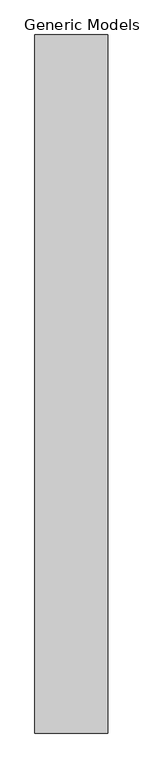
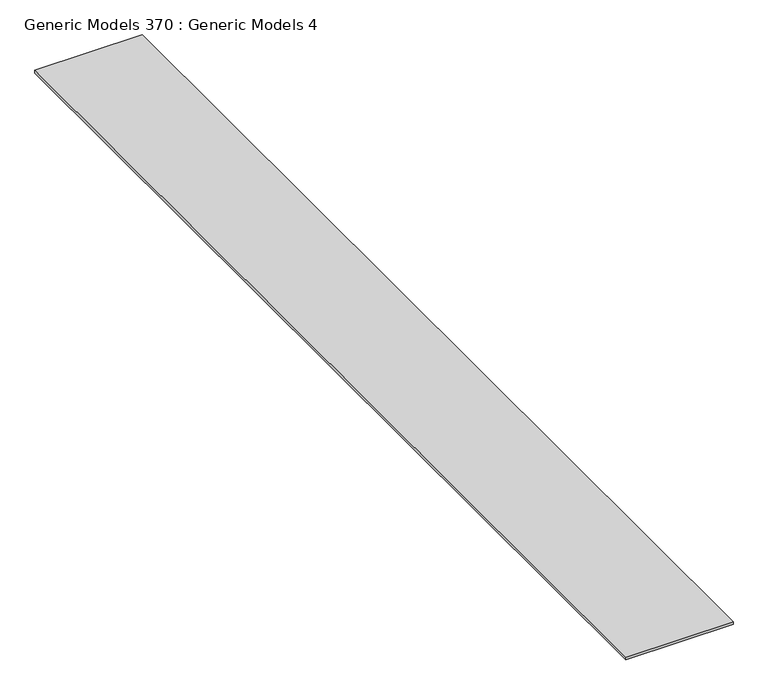
"""IFC4 building model written with IfcOpenShell, lengths in millimetres: proxy geometry, Generic Models 370 : Generic Models 4."""

import ifcopenshell
import ifcopenshell.guid

model = None  # the IFC model being written
_history = None  # IfcOwnerHistory: only IFC2X3 demands one
_inside = {}  # id of a spatial element -> (the spatial element, [elements in it])
_under = {}  # id of a project, library or spatial element -> (it, [spatial elements below it])
_declared = {}  # id of a project -> (the project, [libraries it declares])
_typed = {}  # id of a type object -> (the type object, [elements of that type])
_made_of = {}  # id of a material, layer set ... -> (it, [elements and type objects made of it])


def new_model(schema):
    """Start an empty IFC model of exactly this schema.

    Asked for "IFC4X3", IfcOpenShell would pick the latest addendum, in which some entities
    have other attributes; the version numbers below select the first issue.
    IFC2X3 requires an IfcOwnerHistory on every rooted entity: one is made here for all.
    """
    global model, _history
    if schema == "IFC4X3":
        model = ifcopenshell.file(schema_version=(4, 3, 0, 0))
    else:
        model = ifcopenshell.file(schema=schema)
    _inside.clear()
    _under.clear()
    _declared.clear()
    _typed.clear()
    _made_of.clear()
    _history = None
    if model.schema == "IFC2X3":
        org = make("IfcOrganization", Name="unknown")
        user = make(
            "IfcPersonAndOrganization",
            ThePerson=make("IfcPerson", FamilyName="unknown"),
            TheOrganization=org,
        )
        app = make(
            "IfcApplication",
            ApplicationDeveloper=org,
            Version="unknown",
            ApplicationFullName="unknown",
            ApplicationIdentifier="unknown",
        )
        _history = make(
            "IfcOwnerHistory",
            OwningUser=user,
            OwningApplication=app,
            ChangeAction="ADDED",
            CreationDate=0,
        )
    return model


def make(cls, **values):
    """One entity of the class cls with the attributes given. An attribute that is None is left unset."""
    return model.create_entity(
        cls, **{name: value for name, value in values.items() if value is not None}
    )


def rooted(cls, **values):
    """An entity with a GlobalId (a new one), such as an element, a storey or a relation."""
    return make(cls, GlobalId=ifcopenshell.guid.new(), OwnerHistory=_history, **values)


def si_unit(unit_type, name, prefix=None):
    """IfcSIUnit, for example si_unit("LENGTHUNIT", "METRE", prefix="MILLI")."""
    return make("IfcSIUnit", UnitType=unit_type, Prefix=prefix, Name=name)


def assignment(units):
    """IfcUnitAssignment: the units of a project."""
    return None if units is None else make("IfcUnitAssignment", Units=units)


def point(xyz):
    """IfcCartesianPoint."""
    return None if xyz is None else make("IfcCartesianPoint", Coordinates=xyz)


def direction(xyz):
    """IfcDirection."""
    return None if xyz is None else make("IfcDirection", DirectionRatios=xyz)


def frame(location, z_axis=None, x_axis=None):
    """IfcAxis2Placement3D, a coordinate frame: its origin and axes. An axis left out is left unset."""
    return make(
        "IfcAxis2Placement3D",
        Location=point(location),
        Axis=direction(z_axis),
        RefDirection=direction(x_axis),
    )


def origin():
    """The frame at (0, 0, 0) with its axes left unset."""
    return frame((0.0, 0.0, 0.0))


def place(relative_to, where):
    """IfcLocalPlacement: puts the frame where relative to a parent placement (None: the world)."""
    return make(
        "IfcLocalPlacement", PlacementRelTo=relative_to, RelativePlacement=where
    )


def context(
    kind, dimensions, precision=None, world=None, true_north=None, identifier=None
):
    """IfcGeometricRepresentationContext, for example the 3D "Model" context."""
    return make(
        "IfcGeometricRepresentationContext",
        ContextIdentifier=identifier,
        ContextType=kind,
        CoordinateSpaceDimension=dimensions,
        Precision=precision,
        WorldCoordinateSystem=world,
        TrueNorth=true_north,
    )


def project(units=None, contexts=None):
    """IfcProject with its units and contexts."""
    return rooted(
        "IfcProject",
        Name="project",
        RepresentationContexts=contexts,
        UnitsInContext=assignment(units),
    )


def spatial(cls, under=None, at=None, **own):
    """A site, building, storey or space (cls), placed at a placement, below another one or the project."""
    s = rooted(cls, ObjectPlacement=at, **own)
    if under is not None:
        _under.setdefault(under.id(), (under, []))[1].append(s)
    return s


def polyline(points):
    """IfcPolyline through the points."""
    return make("IfcPolyline", Points=[point(p) for p in points])


def outline(outer, holes=None, kind="AREA"):
    """IfcArbitraryClosedProfileDef: a profile drawn as a closed curve; with holes, ...WithVoids."""
    if holes is None:
        return make("IfcArbitraryClosedProfileDef", ProfileType=kind, OuterCurve=outer)
    return make(
        "IfcArbitraryProfileDefWithVoids",
        ProfileType=kind,
        OuterCurve=outer,
        InnerCurves=holes,
    )


def extrude(swept, where, along, depth):
    """IfcExtrudedAreaSolid: the profile swept, set in the frame where, extruded along a direction by depth."""
    return make(
        "IfcExtrudedAreaSolid",
        SweptArea=swept,
        Position=where,
        ExtrudedDirection=direction(along),
        Depth=depth,
    )


def shape(context_of_items, identifier, shape_type, items):
    """IfcShapeRepresentation: the items that make up one representation, for example the "Body"."""
    return make(
        "IfcShapeRepresentation",
        ContextOfItems=context_of_items,
        RepresentationIdentifier=identifier,
        RepresentationType=shape_type,
        Items=items,
    )


def source(mapping_origin, context_of_items, identifier, shape_type, items):
    """IfcRepresentationMap: a shape defined once, which mapped items show again and again."""
    return make(
        "IfcRepresentationMap",
        MappingOrigin=mapping_origin,
        MappedRepresentation=shape(context_of_items, identifier, shape_type, items),
    )


def transform(
    local_origin,
    x_axis=None,
    y_axis=None,
    z_axis=None,
    scale=None,
    scale2=None,
    scale3=None,
    uniform=True,
):
    """IfcCartesianTransformationOperator3D, or its non-uniform kind. x_axis, y_axis, z_axis: its Axis1, 2, 3."""
    if uniform:
        return make(
            "IfcCartesianTransformationOperator3D",
            Axis1=direction(x_axis),
            Axis2=direction(y_axis),
            LocalOrigin=point(local_origin),
            Scale=scale,
            Axis3=direction(z_axis),
        )
    return make(
        "IfcCartesianTransformationOperator3DnonUniform",
        Axis1=direction(x_axis),
        Axis2=direction(y_axis),
        LocalOrigin=point(local_origin),
        Scale=scale,
        Axis3=direction(z_axis),
        Scale2=scale2,
        Scale3=scale3,
    )


def mapped(mapping_source, mapping_target):
    """IfcMappedItem: shows the shape of a source again, moved by a transform."""
    return make(
        "IfcMappedItem", MappingSource=mapping_source, MappingTarget=mapping_target
    )


def made_of(thing, what):
    """Note that an element or type object is made of a material, layer set ...; save() writes the relation."""
    if what is not None:
        _made_of.setdefault(what.id(), (what, []))[1].append(thing)
    return thing


def element(
    cls,
    number,
    at=None,
    inside=None,
    cuts=None,
    type_object=None,
    material=None,
    context=None,
    identifier="Body",
    shape_type=None,
    held_by="IfcProductDefinitionShape",
    body=None,
    shapes=None,
    **own,
):
    """One element of the class cls, such as IfcWall. Its Tag is "e" and its number.

    at: its placement. inside: the storey or other place that contains it. cuts: it is an
    opening in that element (IfcRelVoidsElement). A single representation is given by context,
    identifier, shape_type and body (its items); several are given by shapes. held_by: the class
    of the entity that holds the representations. save() writes the other relations.
    """
    e = rooted(cls, Tag="e%d" % number, ObjectPlacement=at, **own)
    if body is not None:
        shapes = [shape(context, identifier, shape_type, body)]
    if shapes is not None:
        e.Representation = make(held_by, Representations=shapes)
    if inside is not None:
        _inside.setdefault(inside.id(), (inside, []))[1].append(e)
    if cuts is not None:
        rooted(
            "IfcRelVoidsElement", RelatingBuildingElement=cuts, RelatedOpeningElement=e
        )
    if type_object is not None:
        _typed.setdefault(type_object.id(), (type_object, []))[1].append(e)
    return made_of(e, material)


def aggregate(whole, parts):
    """IfcRelAggregates: a whole, such as a stair, and the parts it consists of."""
    return rooted("IfcRelAggregates", RelatingObject=whole, RelatedObjects=parts)


def save(model, path):
    """Write the relations noted so far, then the file.

    IfcRelAggregates (storeys below a building ...), IfcRelContainedInSpatialStructure (elements
    in a storey), IfcRelDefinesByType, IfcRelAssociatesMaterial and IfcRelDeclares: one each for
    every whole, place, type object, material and project.
    """
    for whole, parts in _under.values():
        aggregate(whole, parts)
    for where, things in _inside.values():
        rooted(
            "IfcRelContainedInSpatialStructure",
            RelatedElements=things,
            RelatingStructure=where,
        )
    for kind, things in _typed.values():
        rooted("IfcRelDefinesByType", RelatedObjects=things, RelatingType=kind)
    for what, things in _made_of.values():
        rooted("IfcRelAssociatesMaterial", RelatedObjects=things, RelatingMaterial=what)
    for by, libraries in _declared.values():
        rooted("IfcRelDeclares", RelatingContext=by, RelatedDefinitions=libraries)
    model.write(path)


def generic_models_370_generic_models_4_c4932353(model_context):
    return source(origin(), model_context, "Body", "SweptSolid", [
        extrude(outline(polyline([(10201.955181, -6864.9230338), (9532.1363263, -6864.9230338), (9532.1363263, -464.1230338), (10201.955181, -464.1230338), (10201.955181, -6864.9230338)])), frame((0.0, 0.0, 128179.3644528), z_axis=(0.0, 0.0, 1.0), x_axis=(1.0, 0.0, 0.0)), (0.0, 0.0, 1.0), 19.05),
    ])


if __name__ == "__main__":
    model = new_model("IFC4")
    model_context = context("Model", 3, world=origin())
    ifc_project = project(units=[si_unit("LENGTHUNIT", "METRE", prefix="MILLI")], contexts=[model_context])
    site = spatial("IfcSite", under=ifc_project)
    building = spatial("IfcBuilding", under=site)
    placement = place(None, origin())
    generic_models_370_generic_models_4_shape = generic_models_370_generic_models_4_c4932353(model_context)
    element("IfcBuildingElementProxy", 1, Name="Generic Models 370 : Generic Models 4", ObjectType="Generic Models 370 : Generic Models 4", at=placement, inside=building, context=model_context, shape_type="MappedRepresentation", body=[
        mapped(generic_models_370_generic_models_4_shape, transform((0.0, 0.0, 0.0), x_axis=(1.0, 0.0, 0.0), y_axis=(0.0, 1.0, 0.0), z_axis=(0.0, 0.0, 1.0))),
    ])
    save(model, "model.ifc")

# Revit data of these elements
# Element 1 (IfcBuildingElementProxy, "Generic Models 370 : Generic Models 4")
#   Materials on its faces: "_CDX PLYWOOD - SEE STRUCT DWGs"
# Materials
#   "_CDX PLYWOOD - SEE STRUCT DWGs": class "Generic", colour RGB 98 75 74, transparency 0, Cost = 0
